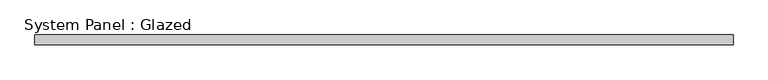
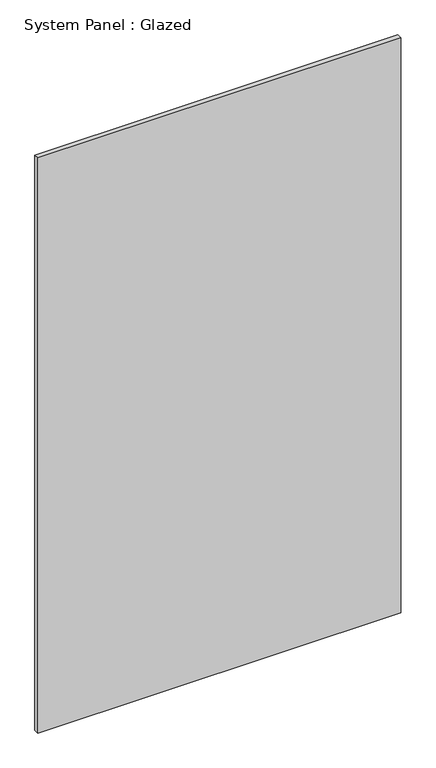
"""IFC4 building model written with IfcOpenShell, lengths in millimetres: plate geometry, System Panel : Glazed."""

import ifcopenshell
import ifcopenshell.guid

model = None  # the IFC model being written
_history = None  # IfcOwnerHistory: only IFC2X3 demands one
_inside = {}  # id of a spatial element -> (the spatial element, [elements in it])
_under = {}  # id of a project, library or spatial element -> (it, [spatial elements below it])
_declared = {}  # id of a project -> (the project, [libraries it declares])
_typed = {}  # id of a type object -> (the type object, [elements of that type])
_made_of = {}  # id of a material, layer set ... -> (it, [elements and type objects made of it])


def new_model(schema):
    """Start an empty IFC model of exactly this schema.

    Asked for "IFC4X3", IfcOpenShell would pick the latest addendum, in which some entities
    have other attributes; the version numbers below select the first issue.
    IFC2X3 requires an IfcOwnerHistory on every rooted entity: one is made here for all.
    """
    global model, _history
    if schema == "IFC4X3":
        model = ifcopenshell.file(schema_version=(4, 3, 0, 0))
    else:
        model = ifcopenshell.file(schema=schema)
    _inside.clear()
    _under.clear()
    _declared.clear()
    _typed.clear()
    _made_of.clear()
    _history = None
    if model.schema == "IFC2X3":
        org = make("IfcOrganization", Name="unknown")
        user = make(
            "IfcPersonAndOrganization",
            ThePerson=make("IfcPerson", FamilyName="unknown"),
            TheOrganization=org,
        )
        app = make(
            "IfcApplication",
            ApplicationDeveloper=org,
            Version="unknown",
            ApplicationFullName="unknown",
            ApplicationIdentifier="unknown",
        )
        _history = make(
            "IfcOwnerHistory",
            OwningUser=user,
            OwningApplication=app,
            ChangeAction="ADDED",
            CreationDate=0,
        )
    return model


def make(cls, **values):
    """One entity of the class cls with the attributes given. An attribute that is None is left unset."""
    return model.create_entity(
        cls, **{name: value for name, value in values.items() if value is not None}
    )


def rooted(cls, **values):
    """An entity with a GlobalId (a new one), such as an element, a storey or a relation."""
    return make(cls, GlobalId=ifcopenshell.guid.new(), OwnerHistory=_history, **values)


def si_unit(unit_type, name, prefix=None):
    """IfcSIUnit, for example si_unit("LENGTHUNIT", "METRE", prefix="MILLI")."""
    return make("IfcSIUnit", UnitType=unit_type, Prefix=prefix, Name=name)


def assignment(units):
    """IfcUnitAssignment: the units of a project."""
    return None if units is None else make("IfcUnitAssignment", Units=units)


def point(xyz):
    """IfcCartesianPoint."""
    return None if xyz is None else make("IfcCartesianPoint", Coordinates=xyz)


def direction(xyz):
    """IfcDirection."""
    return None if xyz is None else make("IfcDirection", DirectionRatios=xyz)


def frame(location, z_axis=None, x_axis=None):
    """IfcAxis2Placement3D, a coordinate frame: its origin and axes. An axis left out is left unset."""
    return make(
        "IfcAxis2Placement3D",
        Location=point(location),
        Axis=direction(z_axis),
        RefDirection=direction(x_axis),
    )


def origin():
    """The frame at (0, 0, 0) with its axes left unset."""
    return frame((0.0, 0.0, 0.0))


def origin_with_axes():
    """The frame at (0, 0, 0) with the z axis (0, 0, 1) and the x axis (1, 0, 0) written out."""
    return frame((0.0, 0.0, 0.0), z_axis=(0.0, 0.0, 1.0), x_axis=(1.0, 0.0, 0.0))


def place(relative_to, where):
    """IfcLocalPlacement: puts the frame where relative to a parent placement (None: the world)."""
    return make(
        "IfcLocalPlacement", PlacementRelTo=relative_to, RelativePlacement=where
    )


def context(
    kind, dimensions, precision=None, world=None, true_north=None, identifier=None
):
    """IfcGeometricRepresentationContext, for example the 3D "Model" context."""
    return make(
        "IfcGeometricRepresentationContext",
        ContextIdentifier=identifier,
        ContextType=kind,
        CoordinateSpaceDimension=dimensions,
        Precision=precision,
        WorldCoordinateSystem=world,
        TrueNorth=true_north,
    )


def project(units=None, contexts=None):
    """IfcProject with its units and contexts."""
    return rooted(
        "IfcProject",
        Name="project",
        RepresentationContexts=contexts,
        UnitsInContext=assignment(units),
    )


def spatial(cls, under=None, at=None, **own):
    """A site, building, storey or space (cls), placed at a placement, below another one or the project."""
    s = rooted(cls, ObjectPlacement=at, **own)
    if under is not None:
        _under.setdefault(under.id(), (under, []))[1].append(s)
    return s


def polyline(points):
    """IfcPolyline through the points."""
    return make("IfcPolyline", Points=[point(p) for p in points])


def outline(outer, holes=None, kind="AREA"):
    """IfcArbitraryClosedProfileDef: a profile drawn as a closed curve; with holes, ...WithVoids."""
    if holes is None:
        return make("IfcArbitraryClosedProfileDef", ProfileType=kind, OuterCurve=outer)
    return make(
        "IfcArbitraryProfileDefWithVoids",
        ProfileType=kind,
        OuterCurve=outer,
        InnerCurves=holes,
    )


def extrude(swept, where, along, depth):
    """IfcExtrudedAreaSolid: the profile swept, set in the frame where, extruded along a direction by depth."""
    return make(
        "IfcExtrudedAreaSolid",
        SweptArea=swept,
        Position=where,
        ExtrudedDirection=direction(along),
        Depth=depth,
    )


def shape(context_of_items, identifier, shape_type, items):
    """IfcShapeRepresentation: the items that make up one representation, for example the "Body"."""
    return make(
        "IfcShapeRepresentation",
        ContextOfItems=context_of_items,
        RepresentationIdentifier=identifier,
        RepresentationType=shape_type,
        Items=items,
    )


def source(mapping_origin, context_of_items, identifier, shape_type, items):
    """IfcRepresentationMap: a shape defined once, which mapped items show again and again."""
    return make(
        "IfcRepresentationMap",
        MappingOrigin=mapping_origin,
        MappedRepresentation=shape(context_of_items, identifier, shape_type, items),
    )


def transform(
    local_origin,
    x_axis=None,
    y_axis=None,
    z_axis=None,
    scale=None,
    scale2=None,
    scale3=None,
    uniform=True,
):
    """IfcCartesianTransformationOperator3D, or its non-uniform kind. x_axis, y_axis, z_axis: its Axis1, 2, 3."""
    if uniform:
        return make(
            "IfcCartesianTransformationOperator3D",
            Axis1=direction(x_axis),
            Axis2=direction(y_axis),
            LocalOrigin=point(local_origin),
            Scale=scale,
            Axis3=direction(z_axis),
        )
    return make(
        "IfcCartesianTransformationOperator3DnonUniform",
        Axis1=direction(x_axis),
        Axis2=direction(y_axis),
        LocalOrigin=point(local_origin),
        Scale=scale,
        Axis3=direction(z_axis),
        Scale2=scale2,
        Scale3=scale3,
    )


def mapped(mapping_source, mapping_target):
    """IfcMappedItem: shows the shape of a source again, moved by a transform."""
    return make(
        "IfcMappedItem", MappingSource=mapping_source, MappingTarget=mapping_target
    )


def made_of(thing, what):
    """Note that an element or type object is made of a material, layer set ...; save() writes the relation."""
    if what is not None:
        _made_of.setdefault(what.id(), (what, []))[1].append(thing)
    return thing


def element(
    cls,
    number,
    at=None,
    inside=None,
    cuts=None,
    type_object=None,
    material=None,
    context=None,
    identifier="Body",
    shape_type=None,
    held_by="IfcProductDefinitionShape",
    body=None,
    shapes=None,
    **own,
):
    """One element of the class cls, such as IfcWall. Its Tag is "e" and its number.

    at: its placement. inside: the storey or other place that contains it. cuts: it is an
    opening in that element (IfcRelVoidsElement). A single representation is given by context,
    identifier, shape_type and body (its items); several are given by shapes. held_by: the class
    of the entity that holds the representations. save() writes the other relations.
    """
    e = rooted(cls, Tag="e%d" % number, ObjectPlacement=at, **own)
    if body is not None:
        shapes = [shape(context, identifier, shape_type, body)]
    if shapes is not None:
        e.Representation = make(held_by, Representations=shapes)
    if inside is not None:
        _inside.setdefault(inside.id(), (inside, []))[1].append(e)
    if cuts is not None:
        rooted(
            "IfcRelVoidsElement", RelatingBuildingElement=cuts, RelatedOpeningElement=e
        )
    if type_object is not None:
        _typed.setdefault(type_object.id(), (type_object, []))[1].append(e)
    return made_of(e, material)


def aggregate(whole, parts):
    """IfcRelAggregates: a whole, such as a stair, and the parts it consists of."""
    return rooted("IfcRelAggregates", RelatingObject=whole, RelatedObjects=parts)


def save(model, path):
    """Write the relations noted so far, then the file.

    IfcRelAggregates (storeys below a building ...), IfcRelContainedInSpatialStructure (elements
    in a storey), IfcRelDefinesByType, IfcRelAssociatesMaterial and IfcRelDeclares: one each for
    every whole, place, type object, material and project.
    """
    for whole, parts in _under.values():
        aggregate(whole, parts)
    for where, things in _inside.values():
        rooted(
            "IfcRelContainedInSpatialStructure",
            RelatedElements=things,
            RelatingStructure=where,
        )
    for kind, things in _typed.values():
        rooted("IfcRelDefinesByType", RelatedObjects=things, RelatingType=kind)
    for what, things in _made_of.values():
        rooted("IfcRelAssociatesMaterial", RelatedObjects=things, RelatingMaterial=what)
    for by, libraries in _declared.values():
        rooted("IfcRelDeclares", RelatingContext=by, RelatedDefinitions=libraries)
    model.write(path)


def system_panel_glazed_35b321d4(model_context):
    return source(origin(), model_context, "Body", "SweptSolid", [
        extrude(outline(polyline([(894.9999998, 24.5), (-894.9999998, 24.5), (-894.9999998, 49.5), (894.9999998, 49.5), (894.9999998, 24.5)])), origin_with_axes(), (0.0, 0.0, 1.0), 3000.0),
    ])


if __name__ == "__main__":
    model = new_model("IFC4")
    model_context = context("Model", 3, world=origin())
    ifc_project = project(units=[si_unit("LENGTHUNIT", "METRE", prefix="MILLI")], contexts=[model_context])
    site = spatial("IfcSite", under=ifc_project)
    building = spatial("IfcBuilding", under=site)
    placement = place(None, origin())
    system_panel_glazed_shape = system_panel_glazed_35b321d4(model_context)
    element("IfcPlate", 1, ObjectType="System Panel : Glazed", at=placement, inside=building, context=model_context, shape_type="MappedRepresentation", body=[
        mapped(system_panel_glazed_shape, transform((0.0, 0.0, 0.0), x_axis=(1.0, 0.0, 0.0), y_axis=(0.0, 1.0, 0.0), z_axis=(0.0, 0.0, 1.0))),
    ])
    save(model, "model.ifc")

# Revit data of these elements
# Type "System Panel : Glazed"
#   Construction Type Id = "GSP4R"
#   Analytic Construction = "1/8 in Pilkington single glazing"
#   Visual Light Transmittance = 0.9
#   Solar Heat Gain Coefficient = 0.86
#   Heat Transfer Coefficient (U) = 6.7069 W/(m²·K)
#   Define Thermal Properties by = 1
# Element 1 (IfcPlate, "System Panel : Glazed")
#   Materials on its faces: "Glass"
# Materials
#   "Glass": class "Glass", colour RGB 0 128 192, transparency 0.9, Description = "Soda Lime Glass", Cost = 0
